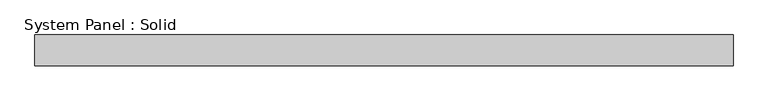
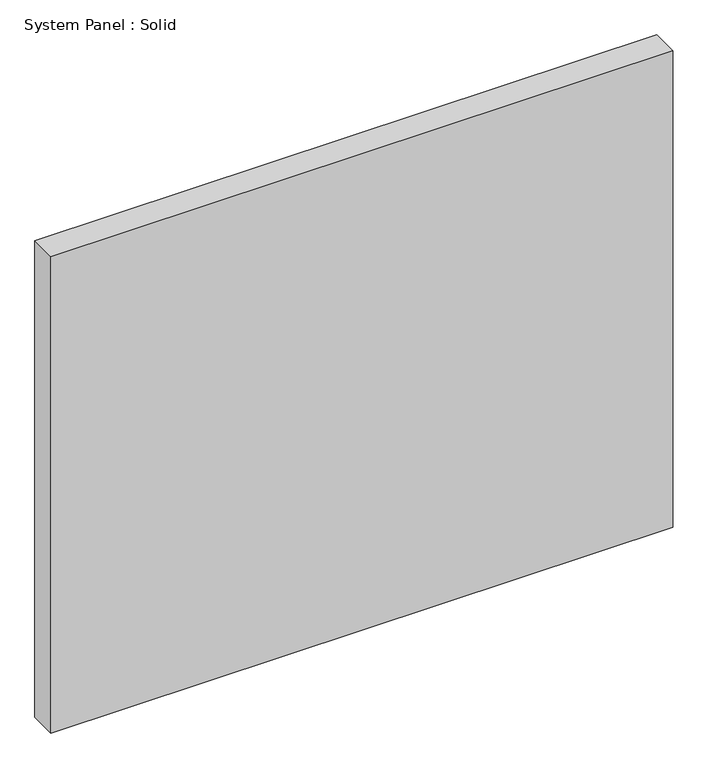
"""IFC4 building model written with IfcOpenShell, lengths in millimetres: plate geometry, System Panel : Solid."""

from ifc_helpers import new_model, si_unit, origin, origin_with_axes, place, context, project, spatial, polyline, outline, extrude, source, transform, mapped, element, save


def system_panel_solid_db88bede(model_context):
    return source(origin(), model_context, "Body", "SweptSolid", [
        extrude(outline(polyline([(713.3166666, -44.45), (-713.3166666, -44.45), (-713.3166666, 19.05), (713.3166666, 19.05), (713.3166666, -44.45)])), origin_with_axes(), (0.0, 0.0, 1.0), 1155.7),
    ])


if __name__ == "__main__":
    model = new_model("IFC4")
    model_context = context("Model", 3, world=origin())
    ifc_project = project(units=[si_unit("LENGTHUNIT", "METRE", prefix="MILLI")], contexts=[model_context])
    site = spatial("IfcSite", under=ifc_project)
    building = spatial("IfcBuilding", under=site)
    placement = place(None, origin())
    system_panel_solid_shape = system_panel_solid_db88bede(model_context)
    element("IfcPlate", 1, ObjectType="System Panel : Solid", at=placement, inside=building, context=model_context, shape_type="MappedRepresentation", body=[
        mapped(system_panel_solid_shape, transform((0.0, 0.0, 0.0), x_axis=(1.0, 0.0, 0.0), y_axis=(0.0, 1.0, 0.0), z_axis=(0.0, 0.0, 1.0))),
    ])
    save(model, "model.ifc")

# Revit data of these elements
# Type "System Panel : Solid"
#   Construction Type Id = "MDOOR"
#   Analytic Construction = "Metal"
#   Visual Light Transmittance = 0
#   Solar Heat Gain Coefficient = 0
#   Heat Transfer Coefficient (U) = 0.651978 BTU/(h·ft²·°F)
#   Define Thermal Properties by = 1
# Element 1 (IfcPlate, "System Panel : Solid")
#   Materials on its faces: "Default"
# Materials
#   "Default": class "Miscellaneous", colour RGB 127 127 127, transparency 0, Cost = 0
